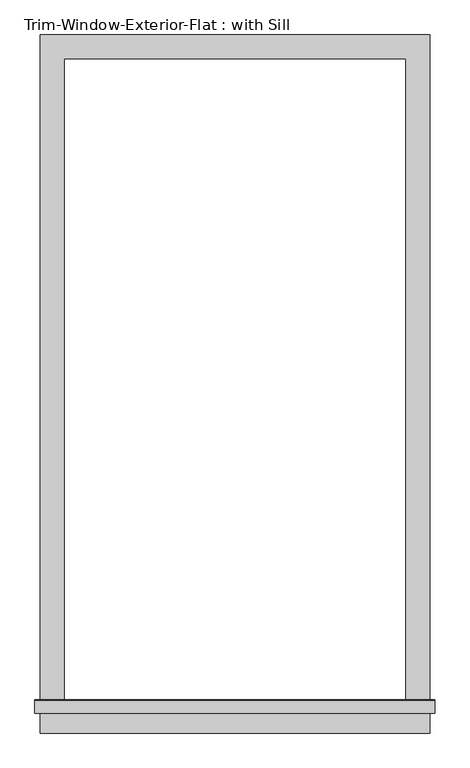
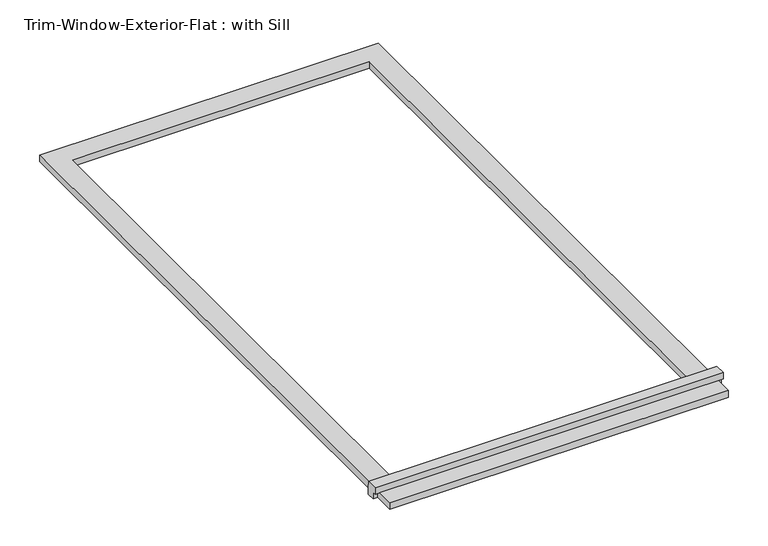
"""IFC4 building model written with IfcOpenShell, lengths in millimetres: proxy geometry, Trim-Window-Exterior-Flat : with Sill."""

from ifc_helpers import new_model, si_unit, frame, origin, origin_with_axes, place, context, project, spatial, polyline, outline, extrude, source, transform, mapped, element, save


def trim_window_exterior_flat_with_sill_994eb4e5(model_context):
    return source(origin(), model_context, "Body", "SweptSolid", [
        extrude(outline(polyline([(463.55, -1546.1823709), (463.55, -1603.3323709), (-463.55, -1603.3323709), (-463.55, -1546.1823709), (463.55, -1546.1823709)])), origin_with_axes(), (0.0, 0.0, 1.0), 19.05),
        extrude(outline(polyline([(-1555.75, 38.1), (-1526.4580645, 38.1), (-1524.0, 19.05), (-1524.0, 0.0), (-1546.1823709, 0.0), (-1546.1823709, 19.05), (-1555.75, 19.05), (-1555.75, 38.1)])), frame((-476.25, 0.0, 0.0), z_axis=(1.0, 0.0, 0.0), x_axis=(0.0, 1.0, 0.0)), (0.0, 0.0, 1.0), 952.5),
        extrude(outline(polyline([(-463.55, 57.15), (463.55, 57.15), (463.55, -1524.0), (406.4, -1524.0), (406.4, 0.0), (-406.4, 0.0), (-406.4, -1524.0), (-463.55, -1524.0), (-463.55, 57.15)])), origin_with_axes(), (0.0, 0.0, 1.0), 19.05),
    ])


if __name__ == "__main__":
    model = new_model("IFC4")
    model_context = context("Model", 3, world=origin())
    ifc_project = project(units=[si_unit("LENGTHUNIT", "METRE", prefix="MILLI")], contexts=[model_context])
    site = spatial("IfcSite", under=ifc_project)
    building = spatial("IfcBuilding", under=site)
    placement = place(None, origin())
    trim_window_exterior_flat_with_sill_shape = trim_window_exterior_flat_with_sill_994eb4e5(model_context)
    element("IfcBuildingElementProxy", 1, Name="Trim-Window-Exterior-Flat : with Sill", ObjectType="Trim-Window-Exterior-Flat : with Sill", at=placement, inside=building, context=model_context, shape_type="MappedRepresentation", body=[
        mapped(trim_window_exterior_flat_with_sill_shape, transform((0.0, 0.0, 0.0), x_axis=(1.0, 0.0, 0.0), y_axis=(0.0, 1.0, 0.0), z_axis=(0.0, 0.0, 1.0))),
    ])
    save(model, "model.ifc")

# Revit data of these elements
# Type "Trim-Window-Exterior-Flat : with Sill"
#   Trim Width = 0' - 2 1/4"
#   Trim Thickness_Picture Frame = 0' - 1 1/4"
#   Trim Thickness_with Sill = 0' - 0 3/4"
#   Sill Thickness = 0' - 1 1/4"
#   Opening Width [instance default] = 2' - 0"
#   Opening Height [instance default] = 3' - 0"
#   Default Elevation = 4' - 0"
#   Sill = yes
#   Picture Frame = no
#   Trim Material [instance default] = none
# Element 1 (IfcBuildingElementProxy, "Trim-Window-Exterior-Flat : with Sill")
#   Opening Width = 2' - 8"
#   Opening Height = 5' - 0"
#   Trim Material = Clad - White
#   Materials on its faces: "Clad - White"
# Materials
#   "Clad - White": class "Wood", colour RGB 242 242 238, transparency 0, Cost = 0
